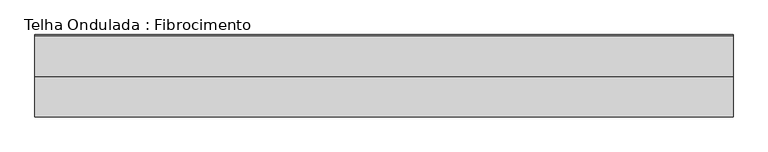
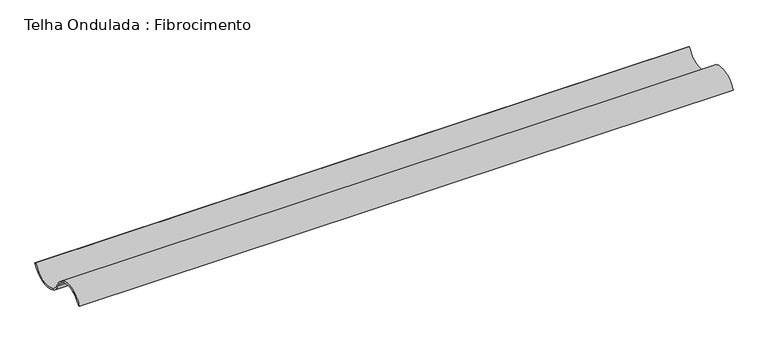
"""IFC4 building model written with IfcOpenShell, lengths in millimetres: beam geometry, Telha Ondulada : Fibrocimento."""

import ifcopenshell
import ifcopenshell.guid

model = None  # the IFC model being written
_history = None  # IfcOwnerHistory: only IFC2X3 demands one
_inside = {}  # id of a spatial element -> (the spatial element, [elements in it])
_under = {}  # id of a project, library or spatial element -> (it, [spatial elements below it])
_declared = {}  # id of a project -> (the project, [libraries it declares])
_typed = {}  # id of a type object -> (the type object, [elements of that type])
_made_of = {}  # id of a material, layer set ... -> (it, [elements and type objects made of it])


def new_model(schema):
    """Start an empty IFC model of exactly this schema.

    Asked for "IFC4X3", IfcOpenShell would pick the latest addendum, in which some entities
    have other attributes; the version numbers below select the first issue.
    IFC2X3 requires an IfcOwnerHistory on every rooted entity: one is made here for all.
    """
    global model, _history
    if schema == "IFC4X3":
        model = ifcopenshell.file(schema_version=(4, 3, 0, 0))
    else:
        model = ifcopenshell.file(schema=schema)
    _inside.clear()
    _under.clear()
    _declared.clear()
    _typed.clear()
    _made_of.clear()
    _history = None
    if model.schema == "IFC2X3":
        org = make("IfcOrganization", Name="unknown")
        user = make(
            "IfcPersonAndOrganization",
            ThePerson=make("IfcPerson", FamilyName="unknown"),
            TheOrganization=org,
        )
        app = make(
            "IfcApplication",
            ApplicationDeveloper=org,
            Version="unknown",
            ApplicationFullName="unknown",
            ApplicationIdentifier="unknown",
        )
        _history = make(
            "IfcOwnerHistory",
            OwningUser=user,
            OwningApplication=app,
            ChangeAction="ADDED",
            CreationDate=0,
        )
    return model


def make(cls, **values):
    """One entity of the class cls with the attributes given. An attribute that is None is left unset."""
    return model.create_entity(
        cls, **{name: value for name, value in values.items() if value is not None}
    )


def rooted(cls, **values):
    """An entity with a GlobalId (a new one), such as an element, a storey or a relation."""
    return make(cls, GlobalId=ifcopenshell.guid.new(), OwnerHistory=_history, **values)


def si_unit(unit_type, name, prefix=None):
    """IfcSIUnit, for example si_unit("LENGTHUNIT", "METRE", prefix="MILLI")."""
    return make("IfcSIUnit", UnitType=unit_type, Prefix=prefix, Name=name)


def assignment(units):
    """IfcUnitAssignment: the units of a project."""
    return None if units is None else make("IfcUnitAssignment", Units=units)


def point(xyz):
    """IfcCartesianPoint."""
    return None if xyz is None else make("IfcCartesianPoint", Coordinates=xyz)


def direction(xyz):
    """IfcDirection."""
    return None if xyz is None else make("IfcDirection", DirectionRatios=xyz)


def frame(location, z_axis=None, x_axis=None):
    """IfcAxis2Placement3D, a coordinate frame: its origin and axes. An axis left out is left unset."""
    return make(
        "IfcAxis2Placement3D",
        Location=point(location),
        Axis=direction(z_axis),
        RefDirection=direction(x_axis),
    )


def frame_2d(location, x_axis=None):
    """IfcAxis2Placement2D, a coordinate frame in the plane: its origin and x axis."""
    return make(
        "IfcAxis2Placement2D", Location=point(location), RefDirection=direction(x_axis)
    )


def origin():
    """The frame at (0, 0, 0) with its axes left unset."""
    return frame((0.0, 0.0, 0.0))


def place(relative_to, where):
    """IfcLocalPlacement: puts the frame where relative to a parent placement (None: the world)."""
    return make(
        "IfcLocalPlacement", PlacementRelTo=relative_to, RelativePlacement=where
    )


def context(
    kind, dimensions, precision=None, world=None, true_north=None, identifier=None
):
    """IfcGeometricRepresentationContext, for example the 3D "Model" context."""
    return make(
        "IfcGeometricRepresentationContext",
        ContextIdentifier=identifier,
        ContextType=kind,
        CoordinateSpaceDimension=dimensions,
        Precision=precision,
        WorldCoordinateSystem=world,
        TrueNorth=true_north,
    )


def project(units=None, contexts=None):
    """IfcProject with its units and contexts."""
    return rooted(
        "IfcProject",
        Name="project",
        RepresentationContexts=contexts,
        UnitsInContext=assignment(units),
    )


def spatial(cls, under=None, at=None, **own):
    """A site, building, storey or space (cls), placed at a placement, below another one or the project."""
    s = rooted(cls, ObjectPlacement=at, **own)
    if under is not None:
        _under.setdefault(under.id(), (under, []))[1].append(s)
    return s


def polyline(points):
    """IfcPolyline through the points."""
    return make("IfcPolyline", Points=[point(p) for p in points])


def circle_curve(where, radius):
    """IfcCircle in the frame where."""
    return make("IfcCircle", Position=where, Radius=radius)


def trimmed(basis, trim1, trim2, sense, master):
    """IfcTrimmedCurve: the piece of a basis curve between two trims."""
    return make(
        "IfcTrimmedCurve",
        BasisCurve=basis,
        Trim1=trim1,
        Trim2=trim2,
        SenseAgreement=sense,
        MasterRepresentation=master,
    )


def segment(curve, same_sense, transition):
    """IfcCompositeCurveSegment."""
    return make(
        "IfcCompositeCurveSegment",
        Transition=transition,
        SameSense=same_sense,
        ParentCurve=curve,
    )


def composite_curve(segments, self_intersect=None):
    """IfcCompositeCurve: segments joined end to end."""
    return make("IfcCompositeCurve", Segments=segments, SelfIntersect=self_intersect)


def outline(outer, holes=None, kind="AREA"):
    """IfcArbitraryClosedProfileDef: a profile drawn as a closed curve; with holes, ...WithVoids."""
    if holes is None:
        return make("IfcArbitraryClosedProfileDef", ProfileType=kind, OuterCurve=outer)
    return make(
        "IfcArbitraryProfileDefWithVoids",
        ProfileType=kind,
        OuterCurve=outer,
        InnerCurves=holes,
    )


def extrude(swept, where, along, depth):
    """IfcExtrudedAreaSolid: the profile swept, set in the frame where, extruded along a direction by depth."""
    return make(
        "IfcExtrudedAreaSolid",
        SweptArea=swept,
        Position=where,
        ExtrudedDirection=direction(along),
        Depth=depth,
    )


def shape(context_of_items, identifier, shape_type, items):
    """IfcShapeRepresentation: the items that make up one representation, for example the "Body"."""
    return make(
        "IfcShapeRepresentation",
        ContextOfItems=context_of_items,
        RepresentationIdentifier=identifier,
        RepresentationType=shape_type,
        Items=items,
    )


def source(mapping_origin, context_of_items, identifier, shape_type, items):
    """IfcRepresentationMap: a shape defined once, which mapped items show again and again."""
    return make(
        "IfcRepresentationMap",
        MappingOrigin=mapping_origin,
        MappedRepresentation=shape(context_of_items, identifier, shape_type, items),
    )


def transform(
    local_origin,
    x_axis=None,
    y_axis=None,
    z_axis=None,
    scale=None,
    scale2=None,
    scale3=None,
    uniform=True,
):
    """IfcCartesianTransformationOperator3D, or its non-uniform kind. x_axis, y_axis, z_axis: its Axis1, 2, 3."""
    if uniform:
        return make(
            "IfcCartesianTransformationOperator3D",
            Axis1=direction(x_axis),
            Axis2=direction(y_axis),
            LocalOrigin=point(local_origin),
            Scale=scale,
            Axis3=direction(z_axis),
        )
    return make(
        "IfcCartesianTransformationOperator3DnonUniform",
        Axis1=direction(x_axis),
        Axis2=direction(y_axis),
        LocalOrigin=point(local_origin),
        Scale=scale,
        Axis3=direction(z_axis),
        Scale2=scale2,
        Scale3=scale3,
    )


def mapped(mapping_source, mapping_target):
    """IfcMappedItem: shows the shape of a source again, moved by a transform."""
    return make(
        "IfcMappedItem", MappingSource=mapping_source, MappingTarget=mapping_target
    )


def made_of(thing, what):
    """Note that an element or type object is made of a material, layer set ...; save() writes the relation."""
    if what is not None:
        _made_of.setdefault(what.id(), (what, []))[1].append(thing)
    return thing


def element(
    cls,
    number,
    at=None,
    inside=None,
    cuts=None,
    type_object=None,
    material=None,
    context=None,
    identifier="Body",
    shape_type=None,
    held_by="IfcProductDefinitionShape",
    body=None,
    shapes=None,
    **own,
):
    """One element of the class cls, such as IfcWall. Its Tag is "e" and its number.

    at: its placement. inside: the storey or other place that contains it. cuts: it is an
    opening in that element (IfcRelVoidsElement). A single representation is given by context,
    identifier, shape_type and body (its items); several are given by shapes. held_by: the class
    of the entity that holds the representations. save() writes the other relations.
    """
    e = rooted(cls, Tag="e%d" % number, ObjectPlacement=at, **own)
    if body is not None:
        shapes = [shape(context, identifier, shape_type, body)]
    if shapes is not None:
        e.Representation = make(held_by, Representations=shapes)
    if inside is not None:
        _inside.setdefault(inside.id(), (inside, []))[1].append(e)
    if cuts is not None:
        rooted(
            "IfcRelVoidsElement", RelatingBuildingElement=cuts, RelatedOpeningElement=e
        )
    if type_object is not None:
        _typed.setdefault(type_object.id(), (type_object, []))[1].append(e)
    return made_of(e, material)


def aggregate(whole, parts):
    """IfcRelAggregates: a whole, such as a stair, and the parts it consists of."""
    return rooted("IfcRelAggregates", RelatingObject=whole, RelatedObjects=parts)


def save(model, path):
    """Write the relations noted so far, then the file.

    IfcRelAggregates (storeys below a building ...), IfcRelContainedInSpatialStructure (elements
    in a storey), IfcRelDefinesByType, IfcRelAssociatesMaterial and IfcRelDeclares: one each for
    every whole, place, type object, material and project.
    """
    for whole, parts in _under.values():
        aggregate(whole, parts)
    for where, things in _inside.values():
        rooted(
            "IfcRelContainedInSpatialStructure",
            RelatedElements=things,
            RelatingStructure=where,
        )
    for kind, things in _typed.values():
        rooted("IfcRelDefinesByType", RelatedObjects=things, RelatingType=kind)
    for what, things in _made_of.values():
        rooted("IfcRelAssociatesMaterial", RelatedObjects=things, RelatingMaterial=what)
    for by, libraries in _declared.values():
        rooted("IfcRelDeclares", RelatingContext=by, RelatedDefinitions=libraries)
    model.write(path)


def telha_ondulada_fibrocimento_69359d52(model_context):
    return source(origin(), model_context, "Body", "SweptSolid", [
        extrude(outline(composite_curve([segment(trimmed(circle_curve(frame_2d((68.3970135, 71.7939461)), 66.7939461), [point((8.3970135, 42.4437972))], [point((128.3970135, 42.4437972))], True, "CARTESIAN"), True, "CONTINUOUS"), segment(polyline([(128.3970135, 42.4437972), (132.8884385, 40.2467307)]), True, "CONTINUOUS"), segment(trimmed(circle_curve(frame_2d((68.3970135, 71.7939461)), 71.7939461), [point((132.8884385, 40.2467307))], [point((3.9055884, 40.2467307))], False, "CARTESIAN"), True, "CONTINUOUS"), segment(trimmed(circle_curve(frame_2d((-51.6029865, 13.0936483)), 61.7939461), [point((3.9055884, 40.2467307))], [point((-107.1115615, 40.2467307))], True, "CARTESIAN"), True, "CONTINUOUS"), segment(polyline([(-107.1115615, 40.2467307), (-111.6029865, 42.4437972)]), True, "CONTINUOUS"), segment(trimmed(circle_curve(frame_2d((-51.6029865, 13.0936483)), 66.7939461), [point((-111.6029865, 42.4437972))], [point((8.3970135, 42.4437972))], False, "CARTESIAN"), True, "CONTINUOUS")], self_intersect=False)), frame((-1038.2805783, 0.0, 0.0), z_axis=(1.0, 0.0, 0.0), x_axis=(0.0, 1.0, 0.0)), (0.0, 0.0, 1.0), 2076.5611566),
    ])


if __name__ == "__main__":
    model = new_model("IFC4")
    model_context = context("Model", 3, world=origin())
    ifc_project = project(units=[si_unit("LENGTHUNIT", "METRE", prefix="MILLI")], contexts=[model_context])
    site = spatial("IfcSite", under=ifc_project)
    building = spatial("IfcBuilding", under=site)
    placement = place(None, origin())
    telha_ondulada_fibrocimento_shape = telha_ondulada_fibrocimento_69359d52(model_context)
    element("IfcBeam", 1, ObjectType="Telha Ondulada : Fibrocimento", at=placement, inside=building, context=model_context, shape_type="MappedRepresentation", body=[
        mapped(telha_ondulada_fibrocimento_shape, transform((0.0, 0.0, 0.0), x_axis=(1.0, 0.0, 0.0), y_axis=(0.0, 1.0, 0.0), z_axis=(0.0, 0.0, 1.0))),
    ])
    save(model, "model.ifc")

# Revit data of these elements
# Type "Telha Ondulada : Fibrocimento"
#   Description = "TELHA ONDULADA FIBROCIMENTO"
#   Cost = 5
#   Length [instance default] = 1.524 m
#   b = 0.07 m
#   h = 0.16 m
#   Structural Material = .TELHA DE FIBROCIMENTO
#   Assembly Code = ""
# Element 1 (IfcBeam, "Telha Ondulada : Fibrocimento")
#   Materials on its faces: ".TELHA DE FIBROCIMENTO"
# Materials
#   ".TELHA DE FIBROCIMENTO": class "CC_TELHADO", colour RGB 77 77 76, transparency 0, Description = "TELHA ONDULADA FIBROCIMENTO", Cost = 0
